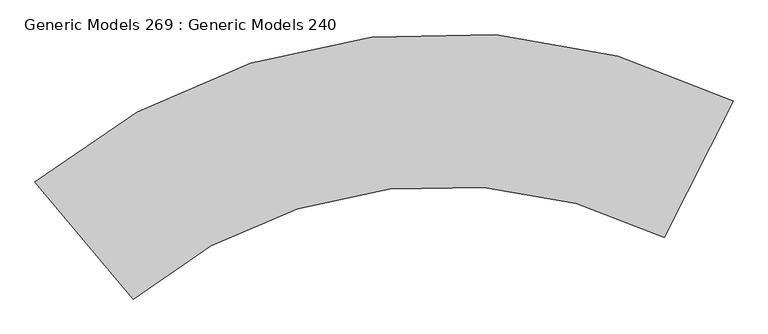
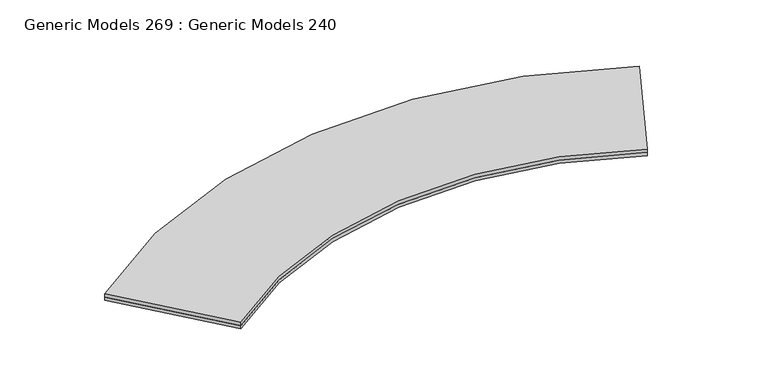
"""IFC4 building model written with IfcOpenShell, lengths in millimetres: proxy geometry, Generic Models 269 : Generic Models 240."""

from ifc_helpers import new_model, si_unit, point, frame, frame_2d, origin, place, context, project, spatial, polyline, circle_curve, trimmed, segment, composite_curve, outline, extrude, source, transform, mapped, element, save


def generic_models_269_generic_models_240_206a0268(model_context):
    return source(origin(), model_context, "Body", "SweptSolid", [
        extrude(outline(composite_curve([segment(trimmed(circle_curve(frame_2d((-832.04683, -25139.2753781)), 2934.2779836), [point((-2715.3785179, -22889.1533729))], [point((485.1270854, -22517.2455991))], False, "CARTESIAN"), True, "CONTINUOUS"), segment(polyline([(485.1270854, -22517.2455991), (170.1471162, -23144.2598827)]), True, "CONTINUOUS"), segment(trimmed(circle_curve(frame_2d((-832.04683, -25139.2753781)), 2232.5947981), [point((170.1471162, -23144.2598827))], [point((-2265.0114479, -23427.2321729))], True, "CARTESIAN"), True, "CONTINUOUS"), segment(polyline([(-2265.0114479, -23427.2321729), (-2715.3785179, -22889.1533729)]), True, "CONTINUOUS")], self_intersect=False)), frame((0.0, 0.0, 781.05), z_axis=(0.0, 0.0, 1.0), x_axis=(1.0, 0.0, 0.0)), (0.0, 0.0, 1.0), 19.05),
        extrude(outline(composite_curve([segment(trimmed(circle_curve(frame_2d((-832.04683, -25139.2753781)), 2934.2779836), [point((-2715.3785179, -22889.1533729))], [point((485.1270854, -22517.2455991))], False, "CARTESIAN"), True, "CONTINUOUS"), segment(polyline([(485.1270854, -22517.2455991), (170.1471162, -23144.2598827)]), True, "CONTINUOUS"), segment(trimmed(circle_curve(frame_2d((-832.04683, -25139.2753781)), 2232.5947981), [point((170.1471162, -23144.2598827))], [point((-2265.0114479, -23427.2321729))], True, "CARTESIAN"), True, "CONTINUOUS"), segment(polyline([(-2265.0114479, -23427.2321729), (-2715.3785179, -22889.1533729)]), True, "CONTINUOUS")], self_intersect=False)), frame((0.0, 0.0, 800.1), z_axis=(0.0, 0.0, 1.0), x_axis=(1.0, 0.0, 0.0)), (0.0, 0.0, 1.0), 19.05),
    ])


if __name__ == "__main__":
    model = new_model("IFC4")
    model_context = context("Model", 3, world=origin())
    ifc_project = project(units=[si_unit("LENGTHUNIT", "METRE", prefix="MILLI")], contexts=[model_context])
    site = spatial("IfcSite", under=ifc_project)
    building = spatial("IfcBuilding", under=site)
    placement = place(None, origin())
    generic_models_269_generic_models_240_shape = generic_models_269_generic_models_240_206a0268(model_context)
    element("IfcBuildingElementProxy", 1, Name="Generic Models 269 : Generic Models 240", ObjectType="Generic Models 269 : Generic Models 240", at=placement, inside=building, context=model_context, shape_type="MappedRepresentation", body=[
        mapped(generic_models_269_generic_models_240_shape, transform((0.0, 0.0, 0.0), x_axis=(1.0, 0.0, 0.0), y_axis=(0.0, 1.0, 0.0), z_axis=(0.0, 0.0, 1.0))),
    ])
    save(model, "model.ifc")

# Revit data of these elements
# Element 1 (IfcBuildingElementProxy, "Generic Models 269 : Generic Models 240")
#   Materials on its faces: "3/4\" PLYWOOD ,GRADE B FINISH (2x)"
# Materials
#   "3/4\" PLYWOOD ,GRADE B FINISH (2x)": class "Wood", colour RGB 48 37 22, transparency 0, Description = "Plywood, sheathing grade", Cost = 0
